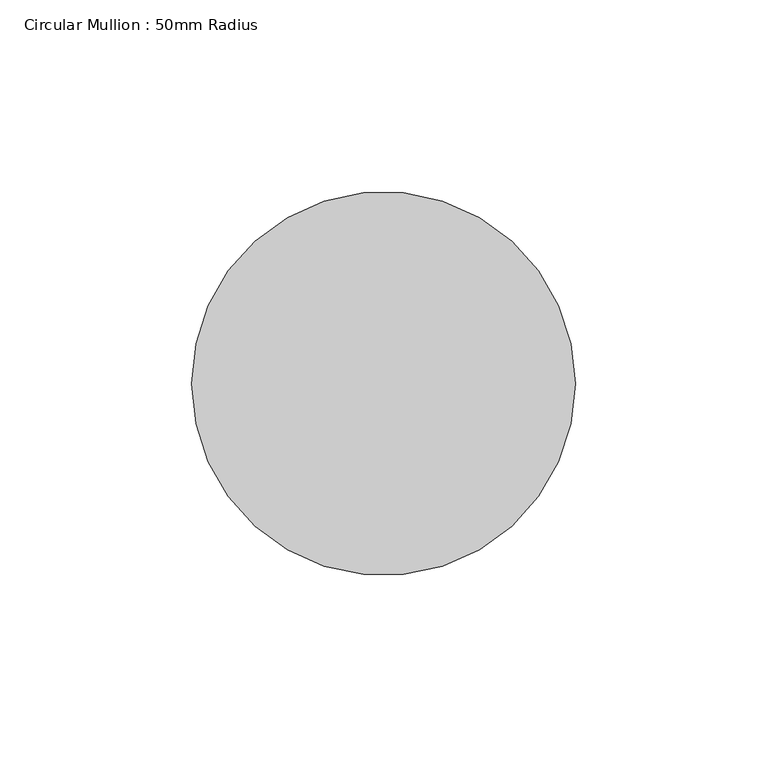
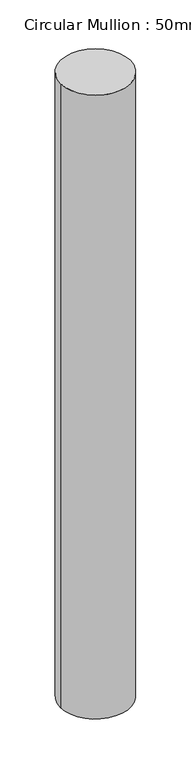
"""IFC4 building model written with IfcOpenShell, lengths in millimetres: member geometry, Circular Mullion : 50mm Radius."""

import ifcopenshell
import ifcopenshell.guid

model = None  # the IFC model being written
_history = None  # IfcOwnerHistory: only IFC2X3 demands one
_inside = {}  # id of a spatial element -> (the spatial element, [elements in it])
_under = {}  # id of a project, library or spatial element -> (it, [spatial elements below it])
_declared = {}  # id of a project -> (the project, [libraries it declares])
_typed = {}  # id of a type object -> (the type object, [elements of that type])
_made_of = {}  # id of a material, layer set ... -> (it, [elements and type objects made of it])


def new_model(schema):
    """Start an empty IFC model of exactly this schema.

    Asked for "IFC4X3", IfcOpenShell would pick the latest addendum, in which some entities
    have other attributes; the version numbers below select the first issue.
    IFC2X3 requires an IfcOwnerHistory on every rooted entity: one is made here for all.
    """
    global model, _history
    if schema == "IFC4X3":
        model = ifcopenshell.file(schema_version=(4, 3, 0, 0))
    else:
        model = ifcopenshell.file(schema=schema)
    _inside.clear()
    _under.clear()
    _declared.clear()
    _typed.clear()
    _made_of.clear()
    _history = None
    if model.schema == "IFC2X3":
        org = make("IfcOrganization", Name="unknown")
        user = make(
            "IfcPersonAndOrganization",
            ThePerson=make("IfcPerson", FamilyName="unknown"),
            TheOrganization=org,
        )
        app = make(
            "IfcApplication",
            ApplicationDeveloper=org,
            Version="unknown",
            ApplicationFullName="unknown",
            ApplicationIdentifier="unknown",
        )
        _history = make(
            "IfcOwnerHistory",
            OwningUser=user,
            OwningApplication=app,
            ChangeAction="ADDED",
            CreationDate=0,
        )
    return model


def make(cls, **values):
    """One entity of the class cls with the attributes given. An attribute that is None is left unset."""
    return model.create_entity(
        cls, **{name: value for name, value in values.items() if value is not None}
    )


def rooted(cls, **values):
    """An entity with a GlobalId (a new one), such as an element, a storey or a relation."""
    return make(cls, GlobalId=ifcopenshell.guid.new(), OwnerHistory=_history, **values)


def si_unit(unit_type, name, prefix=None):
    """IfcSIUnit, for example si_unit("LENGTHUNIT", "METRE", prefix="MILLI")."""
    return make("IfcSIUnit", UnitType=unit_type, Prefix=prefix, Name=name)


def assignment(units):
    """IfcUnitAssignment: the units of a project."""
    return None if units is None else make("IfcUnitAssignment", Units=units)


def point(xyz):
    """IfcCartesianPoint."""
    return None if xyz is None else make("IfcCartesianPoint", Coordinates=xyz)


def direction(xyz):
    """IfcDirection."""
    return None if xyz is None else make("IfcDirection", DirectionRatios=xyz)


def frame(location, z_axis=None, x_axis=None):
    """IfcAxis2Placement3D, a coordinate frame: its origin and axes. An axis left out is left unset."""
    return make(
        "IfcAxis2Placement3D",
        Location=point(location),
        Axis=direction(z_axis),
        RefDirection=direction(x_axis),
    )


def frame_2d(location, x_axis=None):
    """IfcAxis2Placement2D, a coordinate frame in the plane: its origin and x axis."""
    return make(
        "IfcAxis2Placement2D", Location=point(location), RefDirection=direction(x_axis)
    )


def origin():
    """The frame at (0, 0, 0) with its axes left unset."""
    return frame((0.0, 0.0, 0.0))


def origin_2d():
    """The frame at (0, 0) in the plane with its x axis left unset."""
    return frame_2d((0.0, 0.0))


def place(relative_to, where):
    """IfcLocalPlacement: puts the frame where relative to a parent placement (None: the world)."""
    return make(
        "IfcLocalPlacement", PlacementRelTo=relative_to, RelativePlacement=where
    )


def context(
    kind, dimensions, precision=None, world=None, true_north=None, identifier=None
):
    """IfcGeometricRepresentationContext, for example the 3D "Model" context."""
    return make(
        "IfcGeometricRepresentationContext",
        ContextIdentifier=identifier,
        ContextType=kind,
        CoordinateSpaceDimension=dimensions,
        Precision=precision,
        WorldCoordinateSystem=world,
        TrueNorth=true_north,
    )


def project(units=None, contexts=None):
    """IfcProject with its units and contexts."""
    return rooted(
        "IfcProject",
        Name="project",
        RepresentationContexts=contexts,
        UnitsInContext=assignment(units),
    )


def spatial(cls, under=None, at=None, **own):
    """A site, building, storey or space (cls), placed at a placement, below another one or the project."""
    s = rooted(cls, ObjectPlacement=at, **own)
    if under is not None:
        _under.setdefault(under.id(), (under, []))[1].append(s)
    return s


def circle_curve(where, radius):
    """IfcCircle in the frame where."""
    return make("IfcCircle", Position=where, Radius=radius)


def trimmed(basis, trim1, trim2, sense, master):
    """IfcTrimmedCurve: the piece of a basis curve between two trims."""
    return make(
        "IfcTrimmedCurve",
        BasisCurve=basis,
        Trim1=trim1,
        Trim2=trim2,
        SenseAgreement=sense,
        MasterRepresentation=master,
    )


def segment(curve, same_sense, transition):
    """IfcCompositeCurveSegment."""
    return make(
        "IfcCompositeCurveSegment",
        Transition=transition,
        SameSense=same_sense,
        ParentCurve=curve,
    )


def composite_curve(segments, self_intersect=None):
    """IfcCompositeCurve: segments joined end to end."""
    return make("IfcCompositeCurve", Segments=segments, SelfIntersect=self_intersect)


def outline(outer, holes=None, kind="AREA"):
    """IfcArbitraryClosedProfileDef: a profile drawn as a closed curve; with holes, ...WithVoids."""
    if holes is None:
        return make("IfcArbitraryClosedProfileDef", ProfileType=kind, OuterCurve=outer)
    return make(
        "IfcArbitraryProfileDefWithVoids",
        ProfileType=kind,
        OuterCurve=outer,
        InnerCurves=holes,
    )


def extrude(swept, where, along, depth):
    """IfcExtrudedAreaSolid: the profile swept, set in the frame where, extruded along a direction by depth."""
    return make(
        "IfcExtrudedAreaSolid",
        SweptArea=swept,
        Position=where,
        ExtrudedDirection=direction(along),
        Depth=depth,
    )


def shape(context_of_items, identifier, shape_type, items):
    """IfcShapeRepresentation: the items that make up one representation, for example the "Body"."""
    return make(
        "IfcShapeRepresentation",
        ContextOfItems=context_of_items,
        RepresentationIdentifier=identifier,
        RepresentationType=shape_type,
        Items=items,
    )


def source(mapping_origin, context_of_items, identifier, shape_type, items):
    """IfcRepresentationMap: a shape defined once, which mapped items show again and again."""
    return make(
        "IfcRepresentationMap",
        MappingOrigin=mapping_origin,
        MappedRepresentation=shape(context_of_items, identifier, shape_type, items),
    )


def transform(
    local_origin,
    x_axis=None,
    y_axis=None,
    z_axis=None,
    scale=None,
    scale2=None,
    scale3=None,
    uniform=True,
):
    """IfcCartesianTransformationOperator3D, or its non-uniform kind. x_axis, y_axis, z_axis: its Axis1, 2, 3."""
    if uniform:
        return make(
            "IfcCartesianTransformationOperator3D",
            Axis1=direction(x_axis),
            Axis2=direction(y_axis),
            LocalOrigin=point(local_origin),
            Scale=scale,
            Axis3=direction(z_axis),
        )
    return make(
        "IfcCartesianTransformationOperator3DnonUniform",
        Axis1=direction(x_axis),
        Axis2=direction(y_axis),
        LocalOrigin=point(local_origin),
        Scale=scale,
        Axis3=direction(z_axis),
        Scale2=scale2,
        Scale3=scale3,
    )


def mapped(mapping_source, mapping_target):
    """IfcMappedItem: shows the shape of a source again, moved by a transform."""
    return make(
        "IfcMappedItem", MappingSource=mapping_source, MappingTarget=mapping_target
    )


def made_of(thing, what):
    """Note that an element or type object is made of a material, layer set ...; save() writes the relation."""
    if what is not None:
        _made_of.setdefault(what.id(), (what, []))[1].append(thing)
    return thing


def element(
    cls,
    number,
    at=None,
    inside=None,
    cuts=None,
    type_object=None,
    material=None,
    context=None,
    identifier="Body",
    shape_type=None,
    held_by="IfcProductDefinitionShape",
    body=None,
    shapes=None,
    **own,
):
    """One element of the class cls, such as IfcWall. Its Tag is "e" and its number.

    at: its placement. inside: the storey or other place that contains it. cuts: it is an
    opening in that element (IfcRelVoidsElement). A single representation is given by context,
    identifier, shape_type and body (its items); several are given by shapes. held_by: the class
    of the entity that holds the representations. save() writes the other relations.
    """
    e = rooted(cls, Tag="e%d" % number, ObjectPlacement=at, **own)
    if body is not None:
        shapes = [shape(context, identifier, shape_type, body)]
    if shapes is not None:
        e.Representation = make(held_by, Representations=shapes)
    if inside is not None:
        _inside.setdefault(inside.id(), (inside, []))[1].append(e)
    if cuts is not None:
        rooted(
            "IfcRelVoidsElement", RelatingBuildingElement=cuts, RelatedOpeningElement=e
        )
    if type_object is not None:
        _typed.setdefault(type_object.id(), (type_object, []))[1].append(e)
    return made_of(e, material)


def aggregate(whole, parts):
    """IfcRelAggregates: a whole, such as a stair, and the parts it consists of."""
    return rooted("IfcRelAggregates", RelatingObject=whole, RelatedObjects=parts)


def save(model, path):
    """Write the relations noted so far, then the file.

    IfcRelAggregates (storeys below a building ...), IfcRelContainedInSpatialStructure (elements
    in a storey), IfcRelDefinesByType, IfcRelAssociatesMaterial and IfcRelDeclares: one each for
    every whole, place, type object, material and project.
    """
    for whole, parts in _under.values():
        aggregate(whole, parts)
    for where, things in _inside.values():
        rooted(
            "IfcRelContainedInSpatialStructure",
            RelatedElements=things,
            RelatingStructure=where,
        )
    for kind, things in _typed.values():
        rooted("IfcRelDefinesByType", RelatedObjects=things, RelatingType=kind)
    for what, things in _made_of.values():
        rooted("IfcRelAssociatesMaterial", RelatedObjects=things, RelatingMaterial=what)
    for by, libraries in _declared.values():
        rooted("IfcRelDeclares", RelatingContext=by, RelatedDefinitions=libraries)
    model.write(path)


def circular_mullion_50mm_radius_f6ec859c(model_context):
    return source(origin(), model_context, "Body", "SweptSolid", [
        extrude(outline(composite_curve([segment(trimmed(circle_curve(origin_2d(), 50.0), [point((50.0, 0.0))], [point((-50.0, 0.0))], False, "CARTESIAN"), True, "CONTINUOUS"), segment(trimmed(circle_curve(origin_2d(), 50.0), [point((-50.0, 0.0))], [point((50.0, 0.0))], False, "CARTESIAN"), True, "CONTINUOUS")], self_intersect=False)), frame((0.0, 0.0, -942.2734576), z_axis=(0.0, 0.0, 1.0), x_axis=(1.0, 0.0, 0.0)), (0.0, 0.0, 1.0), 942.2734576),
    ])


if __name__ == "__main__":
    model = new_model("IFC4")
    model_context = context("Model", 3, world=origin())
    ifc_project = project(units=[si_unit("LENGTHUNIT", "METRE", prefix="MILLI")], contexts=[model_context])
    site = spatial("IfcSite", under=ifc_project)
    building = spatial("IfcBuilding", under=site)
    placement = place(None, origin())
    circular_mullion_50mm_radius_shape = circular_mullion_50mm_radius_f6ec859c(model_context)
    element("IfcMember", 1, ObjectType="Circular Mullion : 50mm Radius", at=placement, inside=building, context=model_context, shape_type="MappedRepresentation", body=[
        mapped(circular_mullion_50mm_radius_shape, transform((0.0, 0.0, 0.0), x_axis=(1.0, 0.0, 0.0), y_axis=(0.0, 1.0, 0.0), z_axis=(0.0, 0.0, 1.0))),
    ])
    save(model, "model.ifc")

# Revit data of these elements
# Type "Circular Mullion : 50mm Radius"
#   built-in parameter 1007350 = 0.164042 (stored number, unit not read)
# Element 1 (IfcMember, "Circular Mullion : 50mm Radius")
#   Materials on its faces: "Aluminium"
# Materials
#   "Aluminium": class "Metal", colour RGB 247 247 247, transparency 0, Description = "Aluminium 6061", Cost = 0
